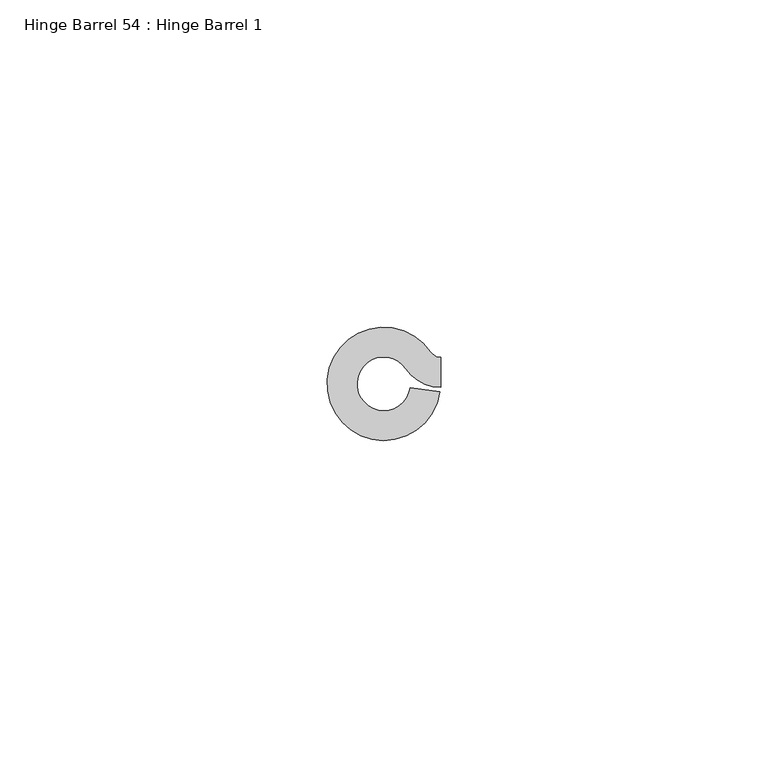
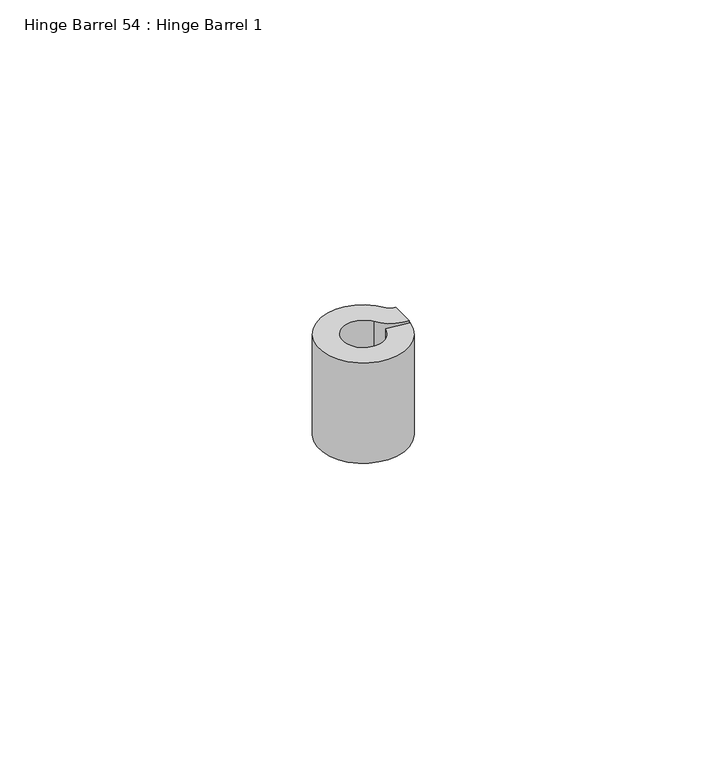
"""IFC4 building model written with IfcOpenShell, lengths in millimetres: proxy geometry, Hinge Barrel 54 : Hinge Barrel 1."""

from ifc_helpers import new_model, si_unit, point, frame, frame_2d, origin, place, context, project, spatial, polyline, circle_curve, trimmed, segment, composite_curve, outline, extrude, source, transform, mapped, element, save


def hinge_barrel_54_hinge_barrel_1_73cfb3f3(model_context):
    return source(origin(), model_context, "Body", "SweptSolid", [
        extrude(outline(composite_curve([segment(trimmed(circle_curve(frame_2d((587319.1320739, -534100.7049841)), 4.0894), [point((587322.5194669, -534098.4139665))], [point((587323.1821338, -534101.2708529))], True, "CARTESIAN"), True, "CONTINUOUS"), segment(polyline([(587323.1821338, -534101.2708529), (587327.7022899, -534101.9024028)]), True, "CONTINUOUS"), segment(trimmed(circle_curve(frame_2d((587319.1320739, -534100.7049841)), 8.6534625), [point((587327.7022899, -534101.9024028))], [point((587326.3000393, -534095.8570273))], False, "CARTESIAN"), True, "CONTINUOUS"), segment(trimmed(circle_curve(frame_2d((587327.8245257, -534094.8259615)), 1.8404226), [point((587326.3000393, -534095.8570273))], [point((587327.8245257, -534096.6663841))], True, "CARTESIAN"), True, "CONTINUOUS"), segment(polyline([(587327.8245257, -534096.6663841), (587327.8245257, -534101.2304466)]), True, "CONTINUOUS"), segment(trimmed(circle_curve(frame_2d((587327.8245257, -534094.8259615)), 6.4044851), [point((587327.8245257, -534101.2304466))], [point((587322.5194669, -534098.4139665))], False, "CARTESIAN"), True, "CONTINUOUS")], self_intersect=False)), frame((0.0, 0.0, 1250.95), z_axis=(0.0, 0.0, 1.0), x_axis=(1.0, 0.0, 0.0)), (0.0, 0.0, 1.0), 20.8359375),
    ])


if __name__ == "__main__":
    model = new_model("IFC4")
    model_context = context("Model", 3, world=origin())
    ifc_project = project(units=[si_unit("LENGTHUNIT", "METRE", prefix="MILLI")], contexts=[model_context])
    site = spatial("IfcSite", under=ifc_project)
    building = spatial("IfcBuilding", under=site)
    placement = place(None, origin())
    hinge_barrel_54_hinge_barrel_1_shape = hinge_barrel_54_hinge_barrel_1_73cfb3f3(model_context)
    element("IfcBuildingElementProxy", 1, Name="Hinge Barrel 54 : Hinge Barrel 1", ObjectType="Hinge Barrel 54 : Hinge Barrel 1", at=placement, inside=building, context=model_context, shape_type="MappedRepresentation", body=[
        mapped(hinge_barrel_54_hinge_barrel_1_shape, transform((0.0, 0.0, 0.0), x_axis=(1.0, 0.0, 0.0), y_axis=(0.0, 1.0, 0.0), z_axis=(0.0, 0.0, 1.0))),
    ])
    save(model, "model.ifc")

# Revit data of these elements
# Element 1 (IfcBuildingElementProxy, "Hinge Barrel 54 : Hinge Barrel 1")
#   Materials on its faces: "6\"X6\" WELD-ON STL BUTT HINGE"
# Materials
#   "6\"X6\" WELD-ON STL BUTT HINGE": class "Metal", colour RGB 189 187 185, transparency 0, Description = "Carbon steel", Cost = 0
